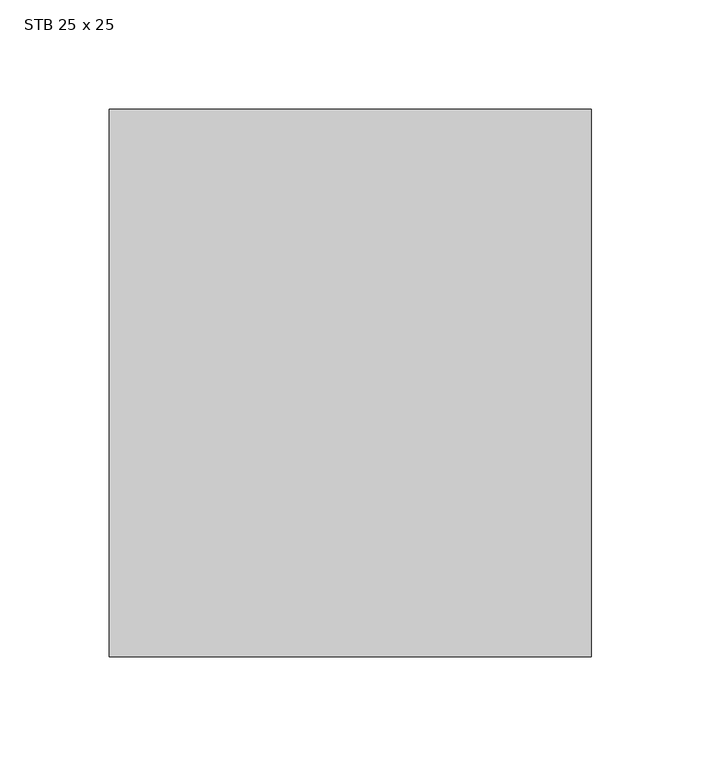
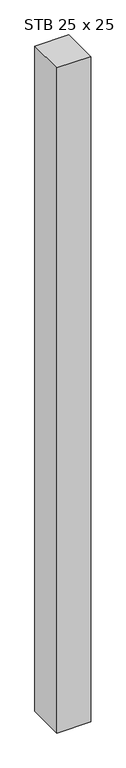
"""IFC4 building model written with IfcOpenShell, lengths in millimetres: column geometry, STB Stütze - rechteckig : STB 25 x 25."""

import ifcopenshell
import ifcopenshell.guid

model = None  # the IFC model being written
_history = None  # IfcOwnerHistory: only IFC2X3 demands one
_inside = {}  # id of a spatial element -> (the spatial element, [elements in it])
_under = {}  # id of a project, library or spatial element -> (it, [spatial elements below it])
_declared = {}  # id of a project -> (the project, [libraries it declares])
_typed = {}  # id of a type object -> (the type object, [elements of that type])
_made_of = {}  # id of a material, layer set ... -> (it, [elements and type objects made of it])


def new_model(schema):
    """Start an empty IFC model of exactly this schema.

    Asked for "IFC4X3", IfcOpenShell would pick the latest addendum, in which some entities
    have other attributes; the version numbers below select the first issue.
    IFC2X3 requires an IfcOwnerHistory on every rooted entity: one is made here for all.
    """
    global model, _history
    if schema == "IFC4X3":
        model = ifcopenshell.file(schema_version=(4, 3, 0, 0))
    else:
        model = ifcopenshell.file(schema=schema)
    _inside.clear()
    _under.clear()
    _declared.clear()
    _typed.clear()
    _made_of.clear()
    _history = None
    if model.schema == "IFC2X3":
        org = make("IfcOrganization", Name="unknown")
        user = make(
            "IfcPersonAndOrganization",
            ThePerson=make("IfcPerson", FamilyName="unknown"),
            TheOrganization=org,
        )
        app = make(
            "IfcApplication",
            ApplicationDeveloper=org,
            Version="unknown",
            ApplicationFullName="unknown",
            ApplicationIdentifier="unknown",
        )
        _history = make(
            "IfcOwnerHistory",
            OwningUser=user,
            OwningApplication=app,
            ChangeAction="ADDED",
            CreationDate=0,
        )
    return model


def make(cls, **values):
    """One entity of the class cls with the attributes given. An attribute that is None is left unset."""
    return model.create_entity(
        cls, **{name: value for name, value in values.items() if value is not None}
    )


def rooted(cls, **values):
    """An entity with a GlobalId (a new one), such as an element, a storey or a relation."""
    return make(cls, GlobalId=ifcopenshell.guid.new(), OwnerHistory=_history, **values)


def si_unit(unit_type, name, prefix=None):
    """IfcSIUnit, for example si_unit("LENGTHUNIT", "METRE", prefix="MILLI")."""
    return make("IfcSIUnit", UnitType=unit_type, Prefix=prefix, Name=name)


def assignment(units):
    """IfcUnitAssignment: the units of a project."""
    return None if units is None else make("IfcUnitAssignment", Units=units)


def point(xyz):
    """IfcCartesianPoint."""
    return None if xyz is None else make("IfcCartesianPoint", Coordinates=xyz)


def direction(xyz):
    """IfcDirection."""
    return None if xyz is None else make("IfcDirection", DirectionRatios=xyz)


def frame(location, z_axis=None, x_axis=None):
    """IfcAxis2Placement3D, a coordinate frame: its origin and axes. An axis left out is left unset."""
    return make(
        "IfcAxis2Placement3D",
        Location=point(location),
        Axis=direction(z_axis),
        RefDirection=direction(x_axis),
    )


def origin():
    """The frame at (0, 0, 0) with its axes left unset."""
    return frame((0.0, 0.0, 0.0))


def place(relative_to, where):
    """IfcLocalPlacement: puts the frame where relative to a parent placement (None: the world)."""
    return make(
        "IfcLocalPlacement", PlacementRelTo=relative_to, RelativePlacement=where
    )


def context(
    kind, dimensions, precision=None, world=None, true_north=None, identifier=None
):
    """IfcGeometricRepresentationContext, for example the 3D "Model" context."""
    return make(
        "IfcGeometricRepresentationContext",
        ContextIdentifier=identifier,
        ContextType=kind,
        CoordinateSpaceDimension=dimensions,
        Precision=precision,
        WorldCoordinateSystem=world,
        TrueNorth=true_north,
    )


def project(units=None, contexts=None):
    """IfcProject with its units and contexts."""
    return rooted(
        "IfcProject",
        Name="project",
        RepresentationContexts=contexts,
        UnitsInContext=assignment(units),
    )


def spatial(cls, under=None, at=None, **own):
    """A site, building, storey or space (cls), placed at a placement, below another one or the project."""
    s = rooted(cls, ObjectPlacement=at, **own)
    if under is not None:
        _under.setdefault(under.id(), (under, []))[1].append(s)
    return s


def polyline(points):
    """IfcPolyline through the points."""
    return make("IfcPolyline", Points=[point(p) for p in points])


def outline(outer, holes=None, kind="AREA"):
    """IfcArbitraryClosedProfileDef: a profile drawn as a closed curve; with holes, ...WithVoids."""
    if holes is None:
        return make("IfcArbitraryClosedProfileDef", ProfileType=kind, OuterCurve=outer)
    return make(
        "IfcArbitraryProfileDefWithVoids",
        ProfileType=kind,
        OuterCurve=outer,
        InnerCurves=holes,
    )


def extrude(swept, where, along, depth):
    """IfcExtrudedAreaSolid: the profile swept, set in the frame where, extruded along a direction by depth."""
    return make(
        "IfcExtrudedAreaSolid",
        SweptArea=swept,
        Position=where,
        ExtrudedDirection=direction(along),
        Depth=depth,
    )


def shape(context_of_items, identifier, shape_type, items):
    """IfcShapeRepresentation: the items that make up one representation, for example the "Body"."""
    return make(
        "IfcShapeRepresentation",
        ContextOfItems=context_of_items,
        RepresentationIdentifier=identifier,
        RepresentationType=shape_type,
        Items=items,
    )


def source(mapping_origin, context_of_items, identifier, shape_type, items):
    """IfcRepresentationMap: a shape defined once, which mapped items show again and again."""
    return make(
        "IfcRepresentationMap",
        MappingOrigin=mapping_origin,
        MappedRepresentation=shape(context_of_items, identifier, shape_type, items),
    )


def transform(
    local_origin,
    x_axis=None,
    y_axis=None,
    z_axis=None,
    scale=None,
    scale2=None,
    scale3=None,
    uniform=True,
):
    """IfcCartesianTransformationOperator3D, or its non-uniform kind. x_axis, y_axis, z_axis: its Axis1, 2, 3."""
    if uniform:
        return make(
            "IfcCartesianTransformationOperator3D",
            Axis1=direction(x_axis),
            Axis2=direction(y_axis),
            LocalOrigin=point(local_origin),
            Scale=scale,
            Axis3=direction(z_axis),
        )
    return make(
        "IfcCartesianTransformationOperator3DnonUniform",
        Axis1=direction(x_axis),
        Axis2=direction(y_axis),
        LocalOrigin=point(local_origin),
        Scale=scale,
        Axis3=direction(z_axis),
        Scale2=scale2,
        Scale3=scale3,
    )


def mapped(mapping_source, mapping_target):
    """IfcMappedItem: shows the shape of a source again, moved by a transform."""
    return make(
        "IfcMappedItem", MappingSource=mapping_source, MappingTarget=mapping_target
    )


def made_of(thing, what):
    """Note that an element or type object is made of a material, layer set ...; save() writes the relation."""
    if what is not None:
        _made_of.setdefault(what.id(), (what, []))[1].append(thing)
    return thing


def element(
    cls,
    number,
    at=None,
    inside=None,
    cuts=None,
    type_object=None,
    material=None,
    context=None,
    identifier="Body",
    shape_type=None,
    held_by="IfcProductDefinitionShape",
    body=None,
    shapes=None,
    **own,
):
    """One element of the class cls, such as IfcWall. Its Tag is "e" and its number.

    at: its placement. inside: the storey or other place that contains it. cuts: it is an
    opening in that element (IfcRelVoidsElement). A single representation is given by context,
    identifier, shape_type and body (its items); several are given by shapes. held_by: the class
    of the entity that holds the representations. save() writes the other relations.
    """
    e = rooted(cls, Tag="e%d" % number, ObjectPlacement=at, **own)
    if body is not None:
        shapes = [shape(context, identifier, shape_type, body)]
    if shapes is not None:
        e.Representation = make(held_by, Representations=shapes)
    if inside is not None:
        _inside.setdefault(inside.id(), (inside, []))[1].append(e)
    if cuts is not None:
        rooted(
            "IfcRelVoidsElement", RelatingBuildingElement=cuts, RelatedOpeningElement=e
        )
    if type_object is not None:
        _typed.setdefault(type_object.id(), (type_object, []))[1].append(e)
    return made_of(e, material)


def aggregate(whole, parts):
    """IfcRelAggregates: a whole, such as a stair, and the parts it consists of."""
    return rooted("IfcRelAggregates", RelatingObject=whole, RelatedObjects=parts)


def save(model, path):
    """Write the relations noted so far, then the file.

    IfcRelAggregates (storeys below a building ...), IfcRelContainedInSpatialStructure (elements
    in a storey), IfcRelDefinesByType, IfcRelAssociatesMaterial and IfcRelDeclares: one each for
    every whole, place, type object, material and project.
    """
    for whole, parts in _under.values():
        aggregate(whole, parts)
    for where, things in _inside.values():
        rooted(
            "IfcRelContainedInSpatialStructure",
            RelatedElements=things,
            RelatingStructure=where,
        )
    for kind, things in _typed.values():
        rooted("IfcRelDefinesByType", RelatedObjects=things, RelatingType=kind)
    for what, things in _made_of.values():
        rooted("IfcRelAssociatesMaterial", RelatedObjects=things, RelatingMaterial=what)
    for by, libraries in _declared.values():
        rooted("IfcRelDeclares", RelatingContext=by, RelatedDefinitions=libraries)
    model.write(path)


def stb_25_x_25_b165da6e(model_context):
    return source(origin(), model_context, "Body", "SweptSolid", [
        extrude(outline(polyline([(110.0, 125.0), (110.0, -125.0), (-110.0, -125.0), (-110.0, 125.0), (110.0, 125.0)])), frame((0.0, 0.0, -1580.0), z_axis=(0.0, 0.0, 1.0), x_axis=(1.0, 0.0, 0.0)), (0.0, 0.0, 1.0), 4600.0),
    ])


if __name__ == "__main__":
    model = new_model("IFC4")
    model_context = context("Model", 3, world=origin())
    ifc_project = project(units=[si_unit("LENGTHUNIT", "METRE", prefix="MILLI")], contexts=[model_context])
    site = spatial("IfcSite", under=ifc_project)
    building = spatial("IfcBuilding", under=site)
    placement = place(None, origin())
    stb_25_x_25_shape = stb_25_x_25_b165da6e(model_context)
    element("IfcColumn", 1, ObjectType="STB Stütze - rechteckig : STB 25 x 25", at=placement, inside=building, context=model_context, shape_type="MappedRepresentation", body=[
        mapped(stb_25_x_25_shape, transform((0.0, 0.0, 0.0), x_axis=(1.0, 0.0, 0.0), y_axis=(0.0, 1.0, 0.0), z_axis=(0.0, 0.0, 1.0))),
    ])
    save(model, "model.ifc")

# Revit data of these elements
# Type "STB Stütze - rechteckig : STB 25 x 25"
#   Breite = 0.220 m
#   Tiefe = 0.250 m
#   Structural Material [instance default] = Stahlbeton - Ortbeton
# Element 1 (IfcColumn, "STB Stütze - rechteckig : STB 25 x 25")
#   Materials on its faces: "Stahlbeton - Ortbeton"
# Materials
#   "Stahlbeton - Ortbeton": class "Beton", colour RGB 247 247 247, transparency 0, Cost = 0
